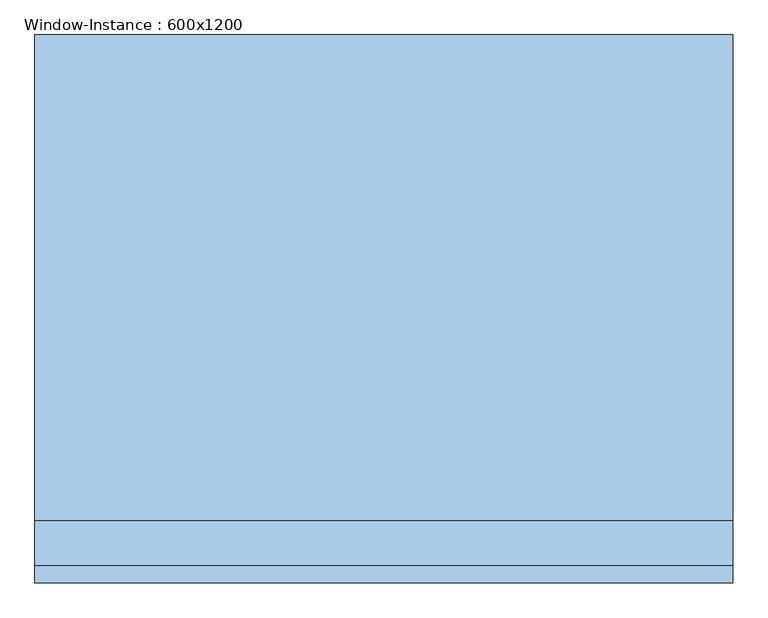
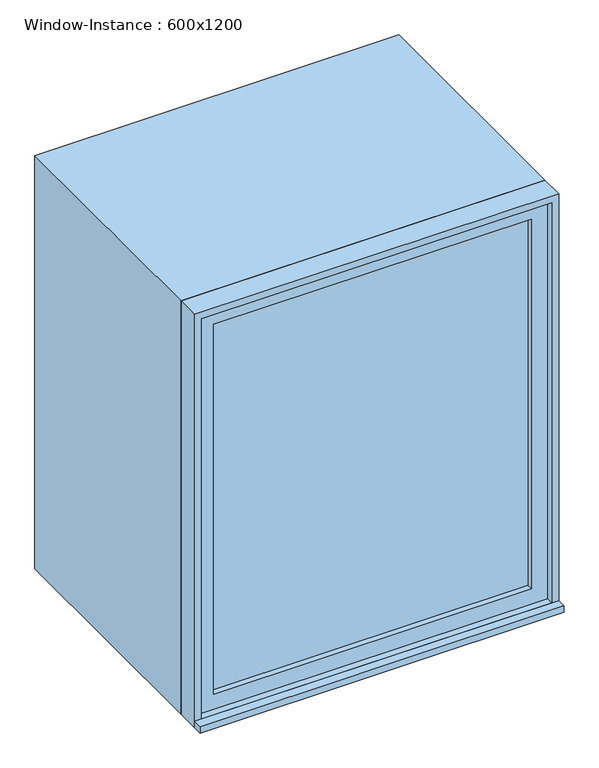
"""IFC4 building model written with IfcOpenShell, lengths in millimetres: window geometry, Window-Instance : 600x1200."""

from ifc_helpers import new_model, si_unit, frame, origin, place, context, project, spatial, polyline, outline, extrude, source, transform, mapped, element, save


def window_instance_600x1200_3ff9373a(model_context):
    return source(origin(), model_context, "Body", "SweptSolid", [
        extrude(outline(polyline([(-538.1, -405.4), (-538.1, -380.0), (461.9, -380.0), (461.9, -405.4), (-538.1, -405.4)])), frame((0.0, 0.0, 900.0), z_axis=(0.0, 0.0, 1.0), x_axis=(1.0, 0.0, 0.0)), (0.0, 0.0, 1.0), 19.05),
        extrude(outline(polyline([(398.4, -331.425), (398.4, -344.125), (-474.6, -344.125), (-474.6, -331.425), (398.4, -331.425)])), frame((0.0, 0.0, 963.5), z_axis=(0.0, 0.0, 1.0), x_axis=(1.0, 0.0, 0.0)), (0.0, 0.0, 1.0), 1073.0),
        extrude(outline(polyline([(2080.95, -519.05), (919.05, -519.05), (919.05, 442.85), (2080.95, 442.85), (2080.95, -519.05)]), holes=[polyline([(2036.5, -474.6), (2036.5, 398.4), (963.5, 398.4), (963.5, -474.6), (2036.5, -474.6)])]), frame((0.0, -360.0, 0.0), z_axis=(0.0, 1.0, 0.0), x_axis=(0.0, 0.0, 1.0)), (0.0, 0.0, 1.0), 44.45),
        extrude(outline(polyline([(2100.0, -538.1), (900.0, -538.1), (900.0, 461.9), (2100.0, 461.9), (2100.0, -538.1)]), holes=[polyline([(2068.25, -506.35), (2068.25, 430.15), (931.75, 430.15), (931.75, -506.35), (2068.25, -506.35)])]), frame((0.0, -315.55, 0.0), z_axis=(0.0, 1.0, 0.0), x_axis=(0.0, 0.0, 1.0)), (0.0, 0.0, 1.0), 695.55),
        extrude(outline(polyline([(2100.0, 461.9), (2100.0, -538.1), (900.0, -538.1), (900.0, 461.9), (2100.0, 461.9)]), holes=[polyline([(2080.95, 442.85), (919.05, 442.85), (919.05, -519.05), (2080.95, -519.05), (2080.95, 442.85)])]), frame((0.0, -380.0, 0.0), z_axis=(0.0, 1.0, 0.0), x_axis=(0.0, 0.0, 1.0)), (0.0, 0.0, 1.0), 64.45),
    ])


if __name__ == "__main__":
    model = new_model("IFC4")
    model_context = context("Model", 3, world=origin())
    ifc_project = project(units=[si_unit("LENGTHUNIT", "METRE", prefix="MILLI")], contexts=[model_context])
    site = spatial("IfcSite", under=ifc_project)
    building = spatial("IfcBuilding", under=site)
    placement = place(None, origin())
    window_instance_600x1200_shape = window_instance_600x1200_3ff9373a(model_context)
    element("IfcWindow", 1, ObjectType="Window-Instance : 600x1200", at=placement, inside=building, context=model_context, shape_type="MappedRepresentation", body=[
        mapped(window_instance_600x1200_shape, transform((0.0, 0.0, 0.0), x_axis=(1.0, 0.0, 0.0), y_axis=(0.0, 1.0, 0.0), z_axis=(0.0, 0.0, 1.0))),
    ])
    save(model, "model.ifc")

# Revit data of these elements
# Type "Window-Instance : 600x1200"
#   Type Mark = "7"
#   Construction Type Id = "GSP4R"
#   Assembly Code = "B2020100"
#   Analytic Construction = "1/8 in Pilkington single glazing"
#   Visual Light Transmittance = 0.9
#   Thermal Resistance (R) = 0.149095 (m²·K)/W
#   Solar Heat Gain Coefficient = 0.86
#   Heat Transfer Coefficient (U) = 6.70716 W/(m²·K)
#   Height [instance default] = 1200 mm
#   Default Sill Height = 900 mm
#   Width [instance default] = 600 mm
#   Window Inset = 20 mm
#   Glass Pane Material = WW-EC-GL-Storefront
#   Sash Material = WW-EC-RGB-White
#   Wall Closure = (empty or 0)
# Element 1 (IfcWindow, "Window-Instance : 600x1200")
#   Width = 1000 mm
#   Materials on its faces: "WW-EC-RGB-White", "WW-EC-GL-Storefront"
# Materials
#   "WW-EC-GL-Storefront": class "Glass", colour RGB 236 240 239, transparency 0.85, Description = "Storefront Glass", Cost = 0
#   "WW-EC-RGB-White": class "Generic", colour RGB 255 255 255, transparency 0, Comments = "If region requests off-white, swith asset color to RGB 231-228-220", Description = "Generic Color", Cost = 0
